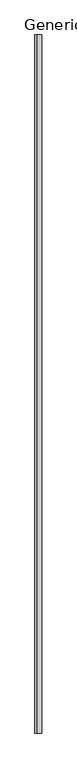
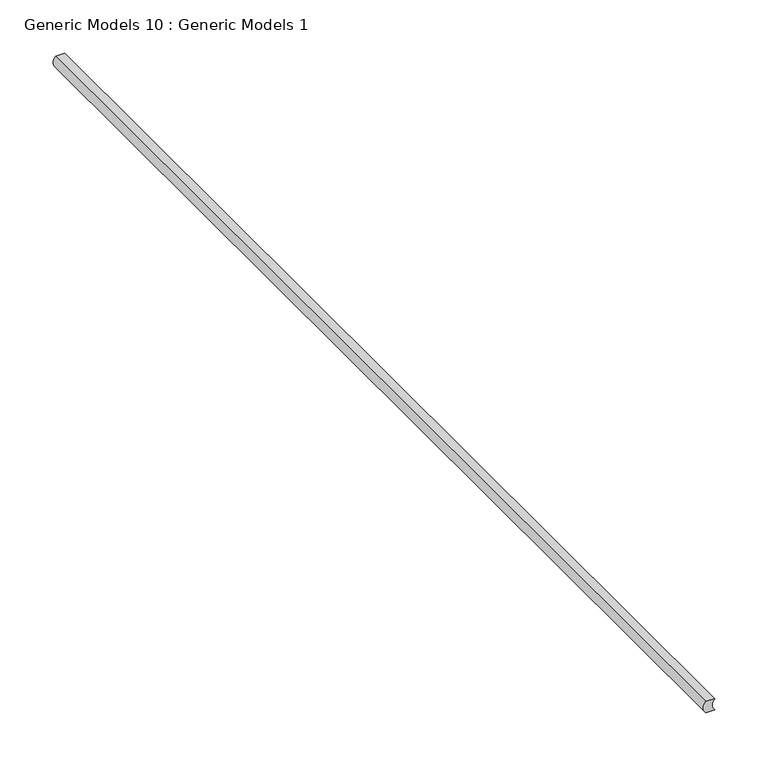
"""IFC4 building model written with IfcOpenShell, lengths in millimetres: proxy geometry, Generic Models 10 : Generic Models 1."""

from ifc_helpers import new_model, si_unit, point, frame, frame_2d, origin, place, context, project, spatial, polyline, circle_curve, trimmed, segment, composite_curve, outline, extrude, source, transform, mapped, element, save


def generic_models_10_generic_models_1_db778090(model_context):
    return source(origin(), model_context, "Body", "SweptSolid", [
        extrude(outline(composite_curve([segment(trimmed(circle_curve(frame_2d((2444.75, 51037.604481)), 8.620055), [point((2438.4, 51031.775))], [point((2451.1, 51031.775))], True, "CARTESIAN"), True, "CONTINUOUS"), segment(polyline([(2451.1, 51031.775), (2451.1, 51022.25)]), True, "CONTINUOUS"), segment(trimmed(circle_curve(frame_2d((2444.75, 51028.079481)), 8.620055), [point((2451.1, 51022.25))], [point((2438.4, 51022.25))], False, "CARTESIAN"), True, "CONTINUOUS"), segment(polyline([(2438.4, 51022.25), (2438.4, 51031.775)]), True, "CONTINUOUS")], self_intersect=False)), frame((0.0, 0.0, 0.0), z_axis=(0.0, 1.0, 0.0), x_axis=(0.0, 0.0, 1.0)), (0.0, 0.0, 1.0), 1219.2),
    ])


if __name__ == "__main__":
    model = new_model("IFC4")
    model_context = context("Model", 3, world=origin())
    ifc_project = project(units=[si_unit("LENGTHUNIT", "METRE", prefix="MILLI")], contexts=[model_context])
    site = spatial("IfcSite", under=ifc_project)
    building = spatial("IfcBuilding", under=site)
    placement = place(None, origin())
    generic_models_10_generic_models_1_shape = generic_models_10_generic_models_1_db778090(model_context)
    element("IfcBuildingElementProxy", 1, Name="Generic Models 10 : Generic Models 1", ObjectType="Generic Models 10 : Generic Models 1", at=placement, inside=building, context=model_context, shape_type="MappedRepresentation", body=[
        mapped(generic_models_10_generic_models_1_shape, transform((0.0, 0.0, 0.0), x_axis=(1.0, 0.0, 0.0), y_axis=(0.0, 1.0, 0.0), z_axis=(0.0, 0.0, 1.0))),
    ])
    save(model, "model.ifc")

# Revit data of these elements
# Element 1 (IfcBuildingElementProxy, "Generic Models 10 : Generic Models 1")
#   Materials on its faces: "ACOUSTICAL SEALANT"
# Materials
#   "ACOUSTICAL SEALANT": class "Unassigned", colour RGB 120 120 120, transparency 0, Cost = 0
